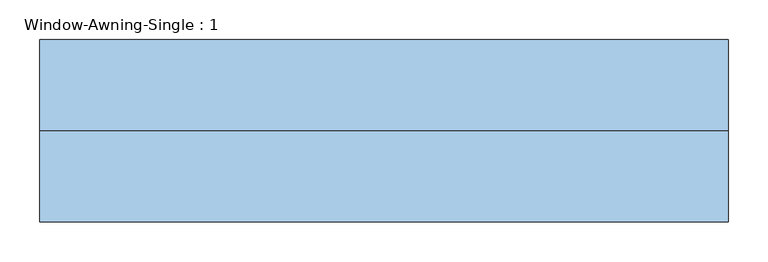
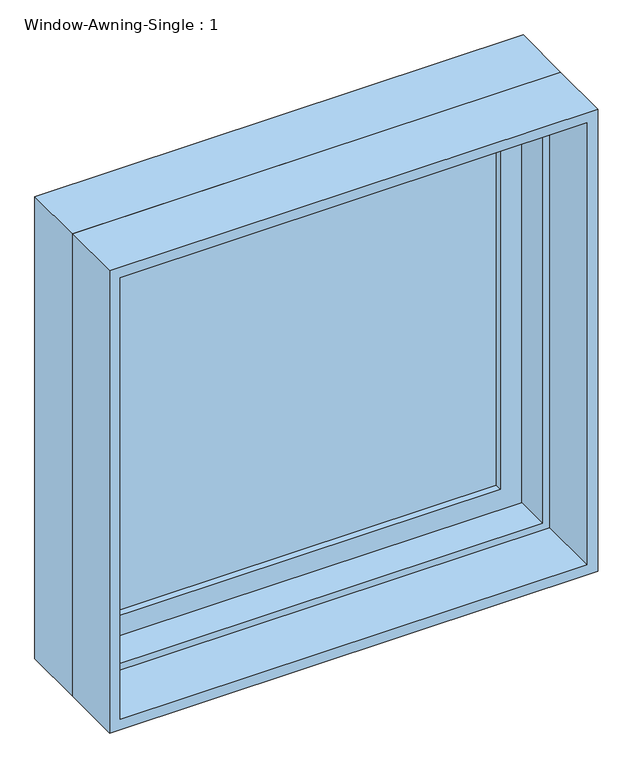
"""IFC4 building model written with IfcOpenShell, lengths in millimetres: window geometry, Window-Awning-Single : 1."""

import ifcopenshell
import ifcopenshell.guid

model = None  # the IFC model being written
_history = None  # IfcOwnerHistory: only IFC2X3 demands one
_inside = {}  # id of a spatial element -> (the spatial element, [elements in it])
_under = {}  # id of a project, library or spatial element -> (it, [spatial elements below it])
_declared = {}  # id of a project -> (the project, [libraries it declares])
_typed = {}  # id of a type object -> (the type object, [elements of that type])
_made_of = {}  # id of a material, layer set ... -> (it, [elements and type objects made of it])


def new_model(schema):
    """Start an empty IFC model of exactly this schema.

    Asked for "IFC4X3", IfcOpenShell would pick the latest addendum, in which some entities
    have other attributes; the version numbers below select the first issue.
    IFC2X3 requires an IfcOwnerHistory on every rooted entity: one is made here for all.
    """
    global model, _history
    if schema == "IFC4X3":
        model = ifcopenshell.file(schema_version=(4, 3, 0, 0))
    else:
        model = ifcopenshell.file(schema=schema)
    _inside.clear()
    _under.clear()
    _declared.clear()
    _typed.clear()
    _made_of.clear()
    _history = None
    if model.schema == "IFC2X3":
        org = make("IfcOrganization", Name="unknown")
        user = make(
            "IfcPersonAndOrganization",
            ThePerson=make("IfcPerson", FamilyName="unknown"),
            TheOrganization=org,
        )
        app = make(
            "IfcApplication",
            ApplicationDeveloper=org,
            Version="unknown",
            ApplicationFullName="unknown",
            ApplicationIdentifier="unknown",
        )
        _history = make(
            "IfcOwnerHistory",
            OwningUser=user,
            OwningApplication=app,
            ChangeAction="ADDED",
            CreationDate=0,
        )
    return model


def make(cls, **values):
    """One entity of the class cls with the attributes given. An attribute that is None is left unset."""
    return model.create_entity(
        cls, **{name: value for name, value in values.items() if value is not None}
    )


def rooted(cls, **values):
    """An entity with a GlobalId (a new one), such as an element, a storey or a relation."""
    return make(cls, GlobalId=ifcopenshell.guid.new(), OwnerHistory=_history, **values)


def si_unit(unit_type, name, prefix=None):
    """IfcSIUnit, for example si_unit("LENGTHUNIT", "METRE", prefix="MILLI")."""
    return make("IfcSIUnit", UnitType=unit_type, Prefix=prefix, Name=name)


def assignment(units):
    """IfcUnitAssignment: the units of a project."""
    return None if units is None else make("IfcUnitAssignment", Units=units)


def point(xyz):
    """IfcCartesianPoint."""
    return None if xyz is None else make("IfcCartesianPoint", Coordinates=xyz)


def direction(xyz):
    """IfcDirection."""
    return None if xyz is None else make("IfcDirection", DirectionRatios=xyz)


def frame(location, z_axis=None, x_axis=None):
    """IfcAxis2Placement3D, a coordinate frame: its origin and axes. An axis left out is left unset."""
    return make(
        "IfcAxis2Placement3D",
        Location=point(location),
        Axis=direction(z_axis),
        RefDirection=direction(x_axis),
    )


def origin():
    """The frame at (0, 0, 0) with its axes left unset."""
    return frame((0.0, 0.0, 0.0))


def place(relative_to, where):
    """IfcLocalPlacement: puts the frame where relative to a parent placement (None: the world)."""
    return make(
        "IfcLocalPlacement", PlacementRelTo=relative_to, RelativePlacement=where
    )


def context(
    kind, dimensions, precision=None, world=None, true_north=None, identifier=None
):
    """IfcGeometricRepresentationContext, for example the 3D "Model" context."""
    return make(
        "IfcGeometricRepresentationContext",
        ContextIdentifier=identifier,
        ContextType=kind,
        CoordinateSpaceDimension=dimensions,
        Precision=precision,
        WorldCoordinateSystem=world,
        TrueNorth=true_north,
    )


def project(units=None, contexts=None):
    """IfcProject with its units and contexts."""
    return rooted(
        "IfcProject",
        Name="project",
        RepresentationContexts=contexts,
        UnitsInContext=assignment(units),
    )


def spatial(cls, under=None, at=None, **own):
    """A site, building, storey or space (cls), placed at a placement, below another one or the project."""
    s = rooted(cls, ObjectPlacement=at, **own)
    if under is not None:
        _under.setdefault(under.id(), (under, []))[1].append(s)
    return s


def polyline(points):
    """IfcPolyline through the points."""
    return make("IfcPolyline", Points=[point(p) for p in points])


def outline(outer, holes=None, kind="AREA"):
    """IfcArbitraryClosedProfileDef: a profile drawn as a closed curve; with holes, ...WithVoids."""
    if holes is None:
        return make("IfcArbitraryClosedProfileDef", ProfileType=kind, OuterCurve=outer)
    return make(
        "IfcArbitraryProfileDefWithVoids",
        ProfileType=kind,
        OuterCurve=outer,
        InnerCurves=holes,
    )


def extrude(swept, where, along, depth):
    """IfcExtrudedAreaSolid: the profile swept, set in the frame where, extruded along a direction by depth."""
    return make(
        "IfcExtrudedAreaSolid",
        SweptArea=swept,
        Position=where,
        ExtrudedDirection=direction(along),
        Depth=depth,
    )


def faces_of(points, faces, orient=None, outer=None):
    """IfcFace entities. A face is a list of loops; a loop is a list of indices into points, from 0.

    orient and outer hold one flag for each loop. By default every Orientation is true, the
    first loop of a face is its IfcFaceOuterBound and the others are IfcFaceBound.
    """
    made = []
    for i, loops in enumerate(faces):
        bounds = []
        for j, loop in enumerate(loops):
            is_outer = j == 0 if outer is None else outer[i][j]
            bounds.append(
                make(
                    "IfcFaceOuterBound" if is_outer else "IfcFaceBound",
                    Bound=make("IfcPolyLoop", Polygon=[points[k] for k in loop]),
                    Orientation=True if orient is None else orient[i][j],
                )
            )
        made.append(make("IfcFace", Bounds=bounds))
    return made


def faceted_brep(points, faces, orient=None, outer=None, voids=None):
    """IfcFacetedBrep: a solid bounded by flat faces; with voids (closed shells), ...WithVoids."""
    shared = [point(p) for p in points]
    hull = make("IfcClosedShell", CfsFaces=faces_of(shared, faces, orient, outer))
    if voids is None:
        return make("IfcFacetedBrep", Outer=hull)
    return make(
        "IfcFacetedBrepWithVoids",
        Outer=hull,
        Voids=[
            make(cls, CfsFaces=faces_of(shared, fs, o, b)) for cls, fs, o, b in voids
        ],
    )


def shape(context_of_items, identifier, shape_type, items):
    """IfcShapeRepresentation: the items that make up one representation, for example the "Body"."""
    return make(
        "IfcShapeRepresentation",
        ContextOfItems=context_of_items,
        RepresentationIdentifier=identifier,
        RepresentationType=shape_type,
        Items=items,
    )


def source(mapping_origin, context_of_items, identifier, shape_type, items):
    """IfcRepresentationMap: a shape defined once, which mapped items show again and again."""
    return make(
        "IfcRepresentationMap",
        MappingOrigin=mapping_origin,
        MappedRepresentation=shape(context_of_items, identifier, shape_type, items),
    )


def transform(
    local_origin,
    x_axis=None,
    y_axis=None,
    z_axis=None,
    scale=None,
    scale2=None,
    scale3=None,
    uniform=True,
):
    """IfcCartesianTransformationOperator3D, or its non-uniform kind. x_axis, y_axis, z_axis: its Axis1, 2, 3."""
    if uniform:
        return make(
            "IfcCartesianTransformationOperator3D",
            Axis1=direction(x_axis),
            Axis2=direction(y_axis),
            LocalOrigin=point(local_origin),
            Scale=scale,
            Axis3=direction(z_axis),
        )
    return make(
        "IfcCartesianTransformationOperator3DnonUniform",
        Axis1=direction(x_axis),
        Axis2=direction(y_axis),
        LocalOrigin=point(local_origin),
        Scale=scale,
        Axis3=direction(z_axis),
        Scale2=scale2,
        Scale3=scale3,
    )


def mapped(mapping_source, mapping_target):
    """IfcMappedItem: shows the shape of a source again, moved by a transform."""
    return make(
        "IfcMappedItem", MappingSource=mapping_source, MappingTarget=mapping_target
    )


def made_of(thing, what):
    """Note that an element or type object is made of a material, layer set ...; save() writes the relation."""
    if what is not None:
        _made_of.setdefault(what.id(), (what, []))[1].append(thing)
    return thing


def element(
    cls,
    number,
    at=None,
    inside=None,
    cuts=None,
    type_object=None,
    material=None,
    context=None,
    identifier="Body",
    shape_type=None,
    held_by="IfcProductDefinitionShape",
    body=None,
    shapes=None,
    **own,
):
    """One element of the class cls, such as IfcWall. Its Tag is "e" and its number.

    at: its placement. inside: the storey or other place that contains it. cuts: it is an
    opening in that element (IfcRelVoidsElement). A single representation is given by context,
    identifier, shape_type and body (its items); several are given by shapes. held_by: the class
    of the entity that holds the representations. save() writes the other relations.
    """
    e = rooted(cls, Tag="e%d" % number, ObjectPlacement=at, **own)
    if body is not None:
        shapes = [shape(context, identifier, shape_type, body)]
    if shapes is not None:
        e.Representation = make(held_by, Representations=shapes)
    if inside is not None:
        _inside.setdefault(inside.id(), (inside, []))[1].append(e)
    if cuts is not None:
        rooted(
            "IfcRelVoidsElement", RelatingBuildingElement=cuts, RelatedOpeningElement=e
        )
    if type_object is not None:
        _typed.setdefault(type_object.id(), (type_object, []))[1].append(e)
    return made_of(e, material)


def aggregate(whole, parts):
    """IfcRelAggregates: a whole, such as a stair, and the parts it consists of."""
    return rooted("IfcRelAggregates", RelatingObject=whole, RelatedObjects=parts)


def save(model, path):
    """Write the relations noted so far, then the file.

    IfcRelAggregates (storeys below a building ...), IfcRelContainedInSpatialStructure (elements
    in a storey), IfcRelDefinesByType, IfcRelAssociatesMaterial and IfcRelDeclares: one each for
    every whole, place, type object, material and project.
    """
    for whole, parts in _under.values():
        aggregate(whole, parts)
    for where, things in _inside.values():
        rooted(
            "IfcRelContainedInSpatialStructure",
            RelatedElements=things,
            RelatingStructure=where,
        )
    for kind, things in _typed.values():
        rooted("IfcRelDefinesByType", RelatedObjects=things, RelatingType=kind)
    for what, things in _made_of.values():
        rooted("IfcRelAssociatesMaterial", RelatedObjects=things, RelatingMaterial=what)
    for by, libraries in _declared.values():
        rooted("IfcRelDeclares", RelatingContext=by, RelatedDefinitions=libraries)
    model.write(path)


def window_awning_single_1_f21cafb6(model_context):
    return source(origin(), model_context, "Body", "SolidModel", [
        faceted_brep([(419.1, 73.025, 927.1), (419.1, 123.825, 927.1), (-419.1, 123.825, 927.1), (-419.1, 73.025, 927.1), (400.05, 9.525, 946.15), (400.05, 73.025, 946.15), (-400.05, 73.025, 946.15), (-400.05, 9.525, 946.15), (431.8, 123.825, 914.4), (431.8, 9.525, 914.4), (-431.8, 9.525, 914.4), (-431.8, 123.825, 914.4), (-419.1, 123.825, 1765.3), (-419.1, 73.025, 1765.3), (-400.05, 73.025, 1746.25), (-400.05, 9.525, 1746.25), (-431.8, 9.525, 1778.0), (-431.8, 123.825, 1778.0), (419.1, 123.825, 1765.3), (419.1, 73.025, 1765.3), (400.05, 73.025, 1746.25), (400.05, 9.525, 1746.25), (431.8, 9.525, 1778.0), (431.8, 123.825, 1778.0)], [[[0, 1, 2, 3]], [[4, 5, 6, 7]], [[8, 9, 10, 11]], [[3, 2, 12, 13]], [[7, 6, 14, 15]], [[11, 10, 16, 17]], [[13, 12, 18, 19]], [[15, 14, 20, 21]], [[17, 16, 22, 23]], [[11, 17, 23, 8], [1, 18, 12, 2]], [[19, 18, 1, 0]], [[3, 13, 19, 0], [5, 20, 14, 6]], [[21, 20, 5, 4]], [[9, 22, 16, 10], [7, 15, 21, 4]], [[23, 22, 9, 8]]]),
        extrude(outline(polyline([(361.95, 104.775), (361.95, 98.425), (-361.95, 98.425), (-361.95, 104.775), (361.95, 104.775)])), frame((0.0, 0.0, 984.25), z_axis=(0.0, 0.0, 1.0), x_axis=(1.0, 0.0, 0.0)), (0.0, 0.0, 1.0), 723.9),
        extrude(outline(polyline([(361.95, 92.075), (361.95, 85.725), (-361.95, 85.725), (-361.95, 92.075), (361.95, 92.075)])), frame((0.0, 0.0, 984.25), z_axis=(0.0, 0.0, 1.0), x_axis=(1.0, 0.0, 0.0)), (0.0, 0.0, 1.0), 723.9),
        extrude(outline(polyline([(927.1, -419.1), (927.1, 419.1), (1765.3, 419.1), (1765.3, -419.1), (927.1, -419.1)]), holes=[polyline([(1708.15, -361.95), (1708.15, 361.95), (984.25, 361.95), (984.25, -361.95), (1708.15, -361.95)])]), frame((0.0, 73.025, 0.0), z_axis=(0.0, 1.0, 0.0), x_axis=(0.0, 0.0, 1.0)), (0.0, 0.0, 1.0), 44.45),
        extrude(outline(polyline([(1778.0, -431.8), (914.4, -431.8), (914.4, 431.8), (1778.0, 431.8), (1778.0, -431.8)]), holes=[polyline([(1758.95, -412.75), (1758.95, 412.75), (933.45, 412.75), (933.45, -412.75), (1758.95, -412.75)])]), frame((0.0, -104.775, 0.0), z_axis=(0.0, 1.0, 0.0), x_axis=(0.0, 0.0, 1.0)), (0.0, 0.0, 1.0), 114.3),
    ])


if __name__ == "__main__":
    model = new_model("IFC4")
    model_context = context("Model", 3, world=origin())
    ifc_project = project(units=[si_unit("LENGTHUNIT", "METRE", prefix="MILLI")], contexts=[model_context])
    site = spatial("IfcSite", under=ifc_project)
    building = spatial("IfcBuilding", under=site)
    placement = place(None, origin())
    window_awning_single_1_shape = window_awning_single_1_f21cafb6(model_context)
    element("IfcWindow", 1, ObjectType="Window-Awning-Single : 1", at=placement, inside=building, context=model_context, shape_type="MappedRepresentation", body=[
        mapped(window_awning_single_1_shape, transform((0.0, 0.0, 0.0), x_axis=(1.0, 0.0, 0.0), y_axis=(0.0, 1.0, 0.0), z_axis=(0.0, 0.0, 1.0))),
    ])
    save(model, "model.ifc")

# Revit data of these elements
# Type "Window-Awning-Single : 1"
#   Type Mark = "18"
#   Fire Rating = "0.5h"
#   Assembly Code = "B2020100"
#   Analytic Construction = "Double glazing - domestic"
#   Window Inset [instance default] = 0' - 0"
#   Wall Thickness [instance default] = 0' - 6"
#   Visual Light Transmittance = 0.81
#   Thermal Resistance (R) = 0.319569 (m²·K)/W
#   Solar Heat Gain Coefficient = 0.76
#   Rough Width = 2' - 10 1/2"
#   Rough Height = 2' - 10 1/2"
#   Interior Wall Closure [instance default] = 0' - 2 1/4"
#   Height = 2' - 10"
#   Heat Transfer Coefficient (U) = 3.12929 W/(m²·K)
#   Frame Extension [instance default] = 0' - 0 1/4"
#   Exterior Wall Closure [instance default] = 0' - 1 1/4"
#   Extension Jamb [instance default] = 0' - 2 1/4"
#   Default Sill Height = 3' - 0"
#   Width = 2' - 10"
#   Muntin Visibility = yes
#   Interior Trim Visibility [instance default] = yes
#   Exterior Trim Visibility [instance default] = yes
#   Extension Jamb Visibility [instance default] = yes
#   Muntin Pattern = Muntin Pattern_2x2 : Muntin Pattern_2x2
#   Interior Trim Material = Wood - Stained
#   Interior Trim = Trim-Window-Interior-Flat : Picture Frame
#   Interior Frame Material = Wood - Stained
#   Glass Panel Material = Glass
#   Exterior Trim Material = Clad - White
#   Exterior Trim = Trim-Window-Exterior-Flat : with Sill
#   Exterior Frame Material = Clad - White
#   Wall Closure = (empty or 0)
# Element 1 (IfcWindow, "Window-Awning-Single : 1")
#   Wall Thickness = 0' - 8 1/4"
#   Extension Jamb = 0' - 4 1/2"
#   Materials on its faces: "Wood - Stained", "Glass", "Clad - White"
# Materials
#   "Wood - Stained": class "Wood", colour RGB 224 178 126, transparency 0, Cost = 0
#   "Glass": class "Glass", colour RGB 218 227 224, transparency 0.85, Description = "Soda Lime Glass", Cost = 0
#   "Clad - White": class "Wood", colour RGB 242 242 238, transparency 0, Cost = 0
